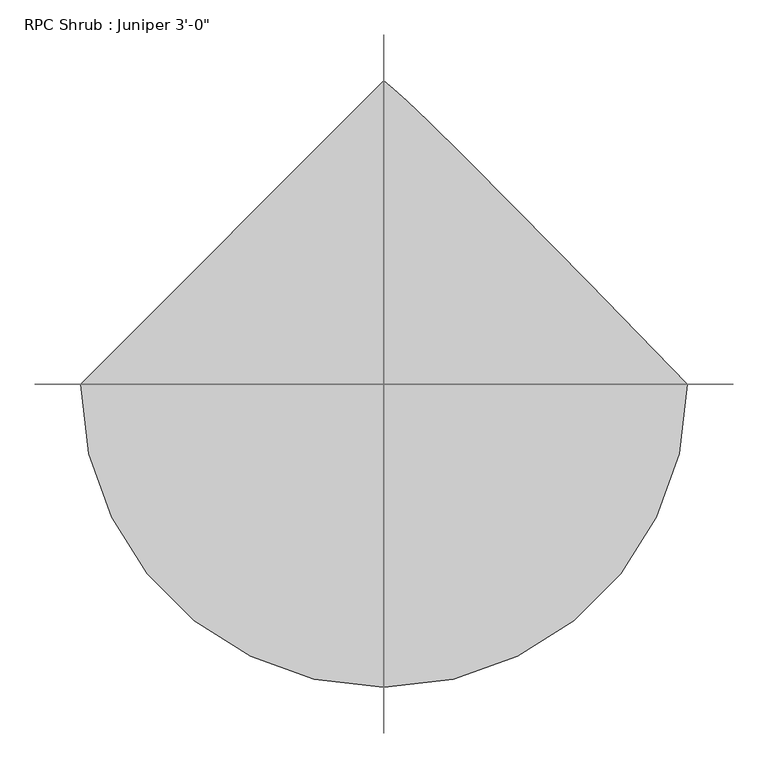
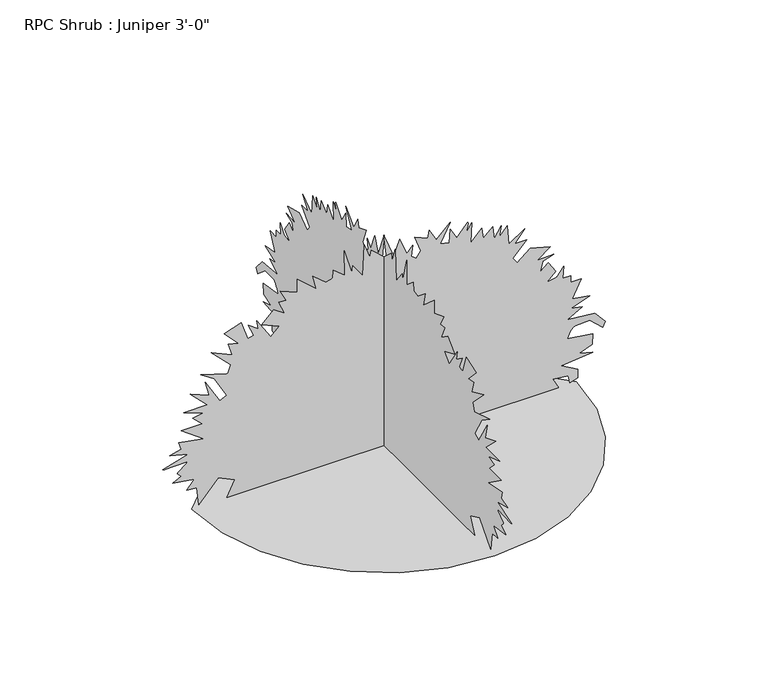
"""IFC4 building model written with IfcOpenShell, lengths in millimetres: geographic element geometry."""

from ifc_helpers import new_model, si_unit, origin, place, context, project, spatial, triangles, source, transform, mapped, element, save


def geographic_element_31b723d7(model_context):
    return source(origin(), model_context, "Body", "Tessellation", [
        triangles([(-789.9406637, 0.0, 7.34e-05), (-769.0593075, -181.0023239, 7.34e-05), (-709.58256, -347.2233553, 7.34e-05), (-616.27561, -493.9033919, 7.34e-05), (-493.9033919, -616.27561, 7.34e-05), (-347.2233553, -709.58256, 7.34e-05), (-181.0023239, -769.0593075, 7.34e-05), (3.45e-05, -789.9406637, 7.34e-05), (181.0025783, -769.0593075, 7.34e-05), (347.2233553, -709.58256, 7.34e-05), (493.9033919, -616.27561, 7.34e-05), (616.27561, -493.9033919, 7.34e-05), (709.58256, -347.2233553, 7.34e-05), (769.0593075, -181.0023239, 7.34e-05), (789.9406637, 6.91e-05, 7.34e-05), (533.2276995, 263.324552, 7.34e-05), (342.9129716, 457.2003633, 7.34e-05), (207.9314215, 593.1996929, 7.34e-05), (117.2157559, 682.8973429, 7.34e-05), (59.6994447, 737.8705862, 7.34e-05), (24.316455, 769.6942978, 7.34e-05), (-0.0001036, 789.9406637, 7.34e-05), (-3.6e-06, -645.975832, 2.9e-06), (1e-06, -614.2334381, 66.8205943), (0.0, -680.8932501, 98.5983058), (0.0, -760.2505428, 9.7171587), (0.0, -769.7755428, 85.9010885), (0.0, -811.0403933, 89.0753315), (0.0, -779.2979994, 127.1672379), (0.0, -868.1777487, 139.8647005), (0.0, -833.2603306, 158.9106491), (0.0, -849.1328356, 174.7823729), (2e-07, -847.0271502, 178.352086), (-1e-07, -810.1082554, 207.9471727), (0.0, -807.8654417, 212.8742702), (2e-07, -903.2958086, 210.5745559), (0.0, -909.4452152, 212.8742702), (0.0, -804.6929609, 244.6174271), (0.0, -880.8752295, 263.6623765), (0.0, -833.2603306, 276.3598392), (0.0, -842.7828598, 308.1047765), (0.0, -741.2056297, 289.0573199), (0.0, -833.2603306, 355.7196754), (0.0, -747.5530621, 355.7196754), (0.0, -785.6455044, 393.8120813), (0.0, -741.2056297, 403.3345379), (0.0, -823.737874, 431.9019439), (0.0, -725.3331247, 431.9019439), (0.0, -795.1679609, 501.7392872), (0.0, -718.9856924, 469.9943499), (0.0, -734.8581247, 533.4817174), (0.0, -674.5432743, 431.9019439), (0.0, -645.975832, 444.5994246), (0.0, -696.7657551, 533.4817174), (0.0, -753.9031105, 571.5741234), (0.0, -642.8008804, 536.6567053), (0.0, -630.1033997, 571.5741234), (0.0, -709.4632359, 650.9314161), (0.0, -623.7558947, 612.8389738), (0.0, -639.6283997, 663.6288969), (0.0, -598.3609694, 654.1063677), (0.0, -655.4982885, 714.4187473), (0.0, -585.663525, 739.8137089), (0.0, -560.2685635, 660.4538727), (0.0, -534.8736382, 666.8038485), (0.0, -557.0935756, 717.5912281), (0.0, -515.8286888, 689.0237858), (6e-07, -522.1761575, 724.2739597), (0.0, -465.0388021, 635.0589111), (0.0, -430.1214203, 669.9763292), (0.0, -503.131208, 701.7212666), (0.0, -452.3413576, 749.3361654), (0.0, -407.901483, 717.5912281), (0.0, -433.2964082, 774.731127), (0.0, -401.5514709, 771.5561028), (0.0, -426.9463961, 819.1710016), (0.0, -357.1115962, 790.6010159), (0.0, -357.1115962, 847.7409147), (0.0, -277.7543035, 777.9035351), (0.0, -293.6242287, 838.2159147), (0.0, -239.6616431, 793.7760401), (0.0, -211.0929654, 800.1260159), (0.0, -207.9182137, 835.043434), (0.0, -160.303333, 796.9510643), (0.0, -163.4780847, 904.8782701), (0.0, -131.7346644, 796.9510643), (0.0, -128.560167, 825.518434), (0.0, -87.2937723, 768.3810785), (0.0, -80.9452954, 901.7032459), (0.0, -58.7248448, 838.2159147), (0.0, -52.3763679, 866.7858278), (0.0, 11.1100709, 809.6484724), (0.0, -1.5869882, 914.4007267), (0.0, 39.6794049, 809.6484724), (0.0, 65.073835, 873.1333328), (0.0, 93.6427671, 800.1260159), (0.0, 119.037447, 828.6934582), (0.0, 112.6887157, 784.2535835), (0.0, 131.7349187, 768.3810785), (0.0, 150.7808674, 793.7760401), (0.0, 125.3861874, 860.4383955), (0.0, 179.3497903, 838.2159147), (0.0, 185.698022, 869.9608521), (0.0, 214.2674628, 819.1710016), (0.0, 271.4042913, 876.308357), (0.0, 230.1389141, 796.9510643), (0.0, 268.2318287, 787.4285351), (0.0, 271.4042913, 844.5658905), (0.0, 299.9742408, 796.9510643), (0.0, 342.3973417, 848.8686802), (0.0, 344.7290671, 848.6756687), (0.0, 345.397086, 844.7309967), (0.0, 338.0666468, 806.4735209), (0.0, 360.2865841, 841.3909389), (0.0, 357.1115962, 755.6835978), (0.0, 401.5540143, 803.2984966), (0.0, 407.901483, 758.858622), (0.0, 445.993889, 793.7760401), (0.0, 452.3413576, 739.8137089), (0.0, 480.9112707, 787.4285351), (0.0, 474.5612949, 739.8137089), (0.0, 506.3062323, 777.9035351), (0.0, 512.6537009, 695.3712908), (0.0, 579.3160563, 739.8137089), (0.0, 538.0486261, 689.0237858), (0.0, 585.663525, 689.0237858), (0.0, 528.5261696, 628.7114788), (0.0, 547.5710827, 603.3165173), (0.0, 601.5359937, 647.7563919), (0.0, 684.0682743, 625.5364546), (0.0, 630.1033997, 584.2716042), (0.0, 696.7657551, 587.4440486), (0.0, 652.3258804, 571.5741234), (0.0, 642.8008804, 530.3066932), (0.0, 674.5458178, 558.8766426), (0.0, 706.2882116, 511.2617801), (0.0, 668.1957693, 476.344362), (0.0, 709.4632359, 482.6918306), (0.0, 738.0306055, 520.7842366), (0.0, 734.8581247, 469.9943499), (0.0, 766.6005186, 469.9943499), (0.0, 766.6005186, 441.4269439), (0.0, 811.0403933, 441.4269439), (0.0, 772.9480236, 368.4171198), (0.0, 845.9578114, 355.7196754), (0.0, 769.7755428, 327.1497259), (0.0, 814.2154175, 317.6272694), (0.0, 753.9031105, 282.7098513), (0.0, 865.0053406, 273.1873765), (0.0, 909.4452152, 222.3972354), (0.0, 899.922686, 200.1767894), (0.0, 845.9578114, 247.7916701), (0.0, 785.3051182, 246.4035645), (0.0, 777.2710882, 242.5165924), (0.0, 770.76618, 236.5473347), (0.0, 765.4803835, 228.9123538), (0.0, 761.1116095, 220.0279215), (0.0, 757.3549347, 210.3106367), (0.0, 753.9031105, 200.1767894), (0.0, 858.6552921, 184.3053381), (0.0, 855.4828114, 139.8647005), (0.0, 801.5179367, 120.8187518), (0.0, 858.6552921, 104.9470462), (0.0, 728.508149, 92.2498288), (0.0, 795.1705044, 54.1576681), (0.0, 795.1705044, 16.0658174), (0.0, 763.4255671, 6.5428419), (0.0, 757.0780621, 38.2862123), (0.0, 693.5907309, 44.6346938), (0.0, 718.9856924, 0.1941814), (-645.975832, 0.000119, 0.0), (-614.2334381, 0.0001104, 66.8205943), (-680.8932501, 0.0001095, 98.5983058), (-760.2505428, 0.0001148, 9.7171587), (-769.7755428, 0.0001102, 85.9010885), (-811.0403933, 0.0001101, 89.0753315), (-779.2979994, 0.0001078, 127.1672379), (-868.1777487, 0.000107, 139.8647005), (-833.2603306, 0.0001059, 158.9106491), (-849.1328356, 0.0001049, 174.7823729), (-847.0271502, 0.0001045, 178.352086), (-810.1082554, 0.000103, 207.9471727), (-807.8654417, 0.0001027, 212.8742702), (-903.2958086, 0.0001026, 210.5745559), (-909.4452152, 0.0001027, 212.8742702), (-804.6929609, 0.0001008, 244.6174271), (-880.8752295, 9.97e-05, 263.6623765), (-833.2603306, 9.89e-05, 276.3598392), (-842.7828598, 9.7e-05, 308.1047765), (-741.2056297, 9.81e-05, 289.0573199), (-833.2603306, 9.42e-05, 355.7196754), (-747.5530621, 9.42e-05, 355.7196754), (-785.6455044, 9.19e-05, 393.8120813), (-741.2056297, 9.13e-05, 403.3345379), (-823.737874, 8.96e-05, 431.9019439), (-725.3331247, 8.96e-05, 431.9019439), (-795.1679609, 8.55e-05, 501.7367437), (-718.9856924, 8.74e-05, 469.9943499), (-734.8581247, 8.36e-05, 533.4817174), (-674.5458178, 8.96e-05, 431.9019439), (-645.975832, 8.89e-05, 444.5994246), (-696.7657551, 8.36e-05, 533.4817174), (-753.9031105, 8.13e-05, 571.5741234), (-642.8008804, 8.34e-05, 536.6567053), (-630.1033997, 8.13e-05, 571.5741234), (-709.4632359, 7.66e-05, 650.9314161), (-623.7558947, 7.88e-05, 612.8389738), (-639.6283997, 7.58e-05, 663.6288969), (-598.3609694, 7.64e-05, 654.1063677), (-655.4982885, 7.28e-05, 714.4187473), (-585.663525, 7.13e-05, 739.8137089), (-560.2685635, 7.6e-05, 660.4538727), (-534.8736382, 7.56e-05, 666.8038485), (-557.0935756, 7.26e-05, 717.5912281), (-515.8286888, 7.43e-05, 689.0237858), (-522.1761575, 7.16e-05, 724.2739597), (-465.0388021, 7.75e-05, 635.0589111), (-430.1214203, 7.54e-05, 669.9763292), (-503.131208, 7.35e-05, 701.7212666), (-452.3413576, 7.07e-05, 749.3361654), (-407.901483, 7.26e-05, 717.5912281), (-433.2964082, 6.92e-05, 774.731127), (-401.5540143, 6.94e-05, 771.5561028), (-426.9463961, 6.65e-05, 819.1710016), (-357.1115962, 6.82e-05, 790.6010159), (-357.1115962, 6.48e-05, 847.7409147), (-277.7543035, 6.9e-05, 777.9035351), (-293.6242287, 6.54e-05, 838.2159147), (-239.6616431, 6.81e-05, 793.7760401), (-211.0929654, 6.77e-05, 800.1260159), (-207.918468, 6.56e-05, 835.043434), (-160.303333, 6.79e-05, 796.9510643), (-163.4780847, 6.14e-05, 904.8782701), (-131.7349187, 6.79e-05, 796.9510643), (-128.560167, 6.62e-05, 825.518434), (-87.2940267, 6.96e-05, 768.3810785), (-80.9452954, 6.16e-05, 901.7032459), (-58.7250992, 6.54e-05, 838.2159147), (-52.3766177, 6.37e-05, 866.7858278), (11.1099687, 6.71e-05, 809.6484724), (-1.5870796, 6.09e-05, 914.4007267), (39.6791505, 6.71e-05, 809.6484724), (65.073835, 6.33e-05, 873.1333328), (93.6427671, 6.77e-05, 800.1260159), (119.037447, 6.6e-05, 828.6934582), (112.6887157, 6.86e-05, 784.2535835), (131.7346644, 6.96e-05, 768.3810785), (150.780613, 6.81e-05, 793.7760401), (125.3861874, 6.41e-05, 860.4358521), (179.349536, 6.54e-05, 838.2159147), (185.698022, 6.35e-05, 869.9608521), (214.2672084, 6.65e-05, 819.1710016), (271.4042913, 6.31e-05, 876.308357), (230.1389141, 6.79e-05, 796.9510643), (268.2318287, 6.84e-05, 787.4285351), (271.4042913, 6.5e-05, 844.5658905), (299.9742408, 6.79e-05, 796.9510643), (342.3973417, 6.48e-05, 848.8686802), (344.7290671, 6.48e-05, 848.6756687), (345.3945425, 6.5e-05, 844.7309967), (338.0666468, 6.73e-05, 806.4735209), (360.2865841, 6.52e-05, 841.3909389), (357.1115962, 7.03e-05, 755.6835978), (401.5514709, 6.75e-05, 803.2984966), (407.901483, 7.01e-05, 758.858622), (445.993889, 6.81e-05, 793.7760401), (452.3413576, 7.13e-05, 739.8137089), (480.9112707, 6.84e-05, 787.4285351), (474.5612949, 7.13e-05, 739.8137089), (506.3062323, 6.9e-05, 777.9035351), (512.6537009, 7.39e-05, 695.3712908), (579.3160563, 7.13e-05, 739.8137089), (538.0486261, 7.43e-05, 689.0237858), (585.663525, 7.43e-05, 689.0237858), (528.5261696, 7.79e-05, 628.7114788), (547.5710827, 7.94e-05, 603.3165173), (601.5359937, 7.68e-05, 647.7563919), (684.0682743, 7.81e-05, 625.5364546), (630.1033997, 8.05e-05, 584.2716042), (696.7657551, 8.04e-05, 587.4440486), (652.3258804, 8.13e-05, 571.5741234), (642.8008804, 8.38e-05, 530.3066932), (674.5458178, 8.21e-05, 558.8766426), (706.2882116, 8.49e-05, 511.2617801), (668.1957693, 8.7e-05, 476.344362), (709.4632359, 8.66e-05, 482.6918306), (738.0306055, 8.43e-05, 520.7842366), (734.8581247, 8.74e-05, 469.9943499), (766.6005186, 8.74e-05, 469.9943499), (766.6005186, 8.91e-05, 441.4269439), (811.0403933, 8.91e-05, 441.4269439), (772.9480236, 9.34e-05, 368.4171198), (845.9578114, 9.42e-05, 355.7196754), (769.7755428, 9.59e-05, 327.1497259), (814.2154175, 9.64e-05, 317.6272694), (753.9031105, 9.85e-05, 282.7098513), (865.0053406, 9.91e-05, 273.1873765), (909.4452152, 0.0001021, 222.3972354), (899.922686, 0.0001034, 200.1767894), (845.9578114, 0.0001006, 247.7916701), (785.3051182, 0.0001007, 246.4035645), (777.2710882, 0.0001009, 242.5165924), (770.76618, 0.0001013, 236.5473347), (765.4803835, 0.0001017, 228.9123538), (761.1116095, 0.0001023, 220.0279215), (757.3549347, 0.0001028, 210.3106367), (753.9031105, 0.0001034, 200.1767894), (858.6552921, 0.0001044, 184.3050838), (855.4828114, 0.000107, 139.8647005), (801.5179367, 0.0001082, 120.8187518), (858.6552921, 0.0001091, 104.9470462), (728.508149, 0.0001099, 92.2495745), (795.1705044, 0.0001121, 54.1576681), (795.1705044, 0.0001144, 16.0658174), (763.4255671, 0.000115, 6.5428419), (757.0780621, 0.0001131, 38.2862123), (693.5907309, 0.0001127, 44.6346938), (718.9856924, 0.0001154, 0.1941786)], [[21, 22, 1], [20, 21, 1], [19, 20, 1], [18, 19, 1], [17, 18, 1], [17, 1, 2], [17, 2, 3], [17, 3, 4], [16, 17, 4], [16, 4, 5], [16, 5, 6], [16, 6, 7], [16, 7, 8], [16, 8, 9], [16, 9, 10], [16, 10, 11], [16, 11, 12], [15, 16, 12], [14, 15, 12], [13, 14, 12], [92, 93, 94], [84, 85, 86], [54, 55, 56], [50, 51, 52], [131, 132, 133], [123, 124, 125], [104, 105, 106], [46, 47, 48], [57, 58, 59], [88, 89, 90], [48, 49, 50], [67, 68, 69], [119, 120, 121], [162, 163, 164], [38, 39, 40], [113, 114, 115], [144, 145, 146], [65, 66, 67], [138, 139, 140], [96, 97, 98], [107, 108, 109], [79, 80, 81], [42, 43, 44], [29, 30, 31], [36, 37, 38], [75, 76, 77], [102, 103, 104], [146, 147, 148], [86, 87, 88], [94, 95, 96], [121, 122, 123], [125, 126, 127], [100, 101, 102], [77, 78, 79], [25, 26, 27], [115, 116, 117], [129, 130, 131], [117, 118, 119], [27, 28, 29], [82, 83, 84], [44, 45, 46], [48, 50, 52], [59, 60, 61], [169, 170, 23], [73, 74, 75], [90, 91, 92], [142, 143, 144], [40, 41, 42], [38, 40, 42], [169, 23, 24], [53, 54, 56], [61, 62, 63], [61, 63, 64], [70, 71, 72], [70, 72, 73], [150, 151, 152], [149, 150, 152], [148, 149, 152], [148, 152, 153], [128, 129, 131], [148, 153, 154], [35, 36, 38], [134, 135, 136], [134, 136, 137], [65, 67, 69], [166, 167, 168], [165, 166, 168], [164, 165, 168], [164, 168, 169], [88, 90, 92], [140, 141, 142], [100, 102, 104], [159, 160, 161], [159, 161, 162], [25, 27, 29], [123, 125, 127], [148, 154, 155], [100, 104, 106], [110, 111, 112], [109, 110, 112], [109, 112, 113], [109, 113, 115], [31, 32, 33], [131, 133, 134], [159, 162, 164], [128, 131, 134], [46, 48, 52], [73, 75, 77], [73, 77, 79], [29, 31, 33], [29, 33, 34], [44, 46, 52], [148, 155, 156], [164, 169, 24], [159, 164, 24], [158, 159, 24], [157, 158, 24], [156, 157, 24], [148, 156, 24], [146, 148, 24], [144, 146, 24], [142, 144, 24], [140, 142, 24], [138, 140, 24], [137, 138, 24], [134, 137, 24], [128, 134, 24], [127, 128, 24], [123, 127, 24], [121, 123, 24], [119, 121, 24], [117, 119, 24], [115, 117, 24], [109, 115, 24], [107, 109, 24], [106, 107, 24], [106, 24, 25], [106, 25, 29], [106, 29, 34], [106, 34, 35], [106, 35, 38], [106, 38, 42], [106, 42, 44], [106, 44, 52], [106, 52, 53], [106, 53, 56], [99, 100, 106], [99, 106, 56], [99, 56, 57], [98, 99, 57], [96, 98, 57], [94, 96, 57], [59, 61, 64], [57, 59, 64], [70, 73, 79], [64, 65, 69], [57, 64, 69], [94, 57, 69], [84, 86, 88], [88, 92, 94], [88, 94, 69], [88, 69, 70], [88, 70, 79], [84, 88, 79], [82, 84, 79], [82, 79, 81], [240, 241, 242], [232, 233, 234], [202, 203, 204], [198, 199, 200], [279, 280, 281], [271, 272, 273], [252, 253, 254], [194, 195, 196], [205, 206, 207], [236, 237, 238], [196, 197, 198], [215, 216, 217], [267, 268, 269], [310, 311, 312], [186, 187, 188], [261, 262, 263], [292, 293, 294], [213, 214, 215], [286, 287, 288], [244, 245, 246], [255, 256, 257], [227, 228, 229], [190, 191, 192], [177, 178, 179], [184, 185, 186], [223, 224, 225], [250, 251, 252], [294, 295, 296], [234, 235, 236], [242, 243, 244], [269, 270, 271], [273, 274, 275], [248, 249, 250], [225, 226, 227], [173, 174, 175], [263, 264, 265], [277, 278, 279], [265, 266, 267], [175, 176, 177], [230, 231, 232], [192, 193, 194], [196, 198, 200], [207, 208, 209], [317, 318, 171], [221, 222, 223], [238, 239, 240], [290, 291, 292], [188, 189, 190], [186, 188, 190], [317, 171, 172], [201, 202, 204], [209, 210, 211], [209, 211, 212], [218, 219, 220], [218, 220, 221], [298, 299, 300], [297, 298, 300], [296, 297, 300], [296, 300, 301], [276, 277, 279], [296, 301, 302], [183, 184, 186], [282, 283, 284], [282, 284, 285], [213, 215, 217], [314, 315, 316], [313, 314, 316], [312, 313, 316], [312, 316, 317], [236, 238, 240], [288, 289, 290], [248, 250, 252], [307, 308, 309], [307, 309, 310], [173, 175, 177], [271, 273, 275], [296, 302, 303], [248, 252, 254], [258, 259, 260], [257, 258, 260], [257, 260, 261], [257, 261, 263], [179, 180, 181], [279, 281, 282], [307, 310, 312], [276, 279, 282], [194, 196, 200], [221, 223, 225], [221, 225, 227], [177, 179, 181], [177, 181, 182], [192, 194, 200], [296, 303, 304], [312, 317, 172], [307, 312, 172], [306, 307, 172], [305, 306, 172], [304, 305, 172], [296, 304, 172], [294, 296, 172], [292, 294, 172], [290, 292, 172], [288, 290, 172], [286, 288, 172], [285, 286, 172], [282, 285, 172], [276, 282, 172], [275, 276, 172], [271, 275, 172], [269, 271, 172], [267, 269, 172], [265, 267, 172], [263, 265, 172], [257, 263, 172], [255, 257, 172], [254, 255, 172], [254, 172, 173], [254, 173, 177], [254, 177, 182], [254, 182, 183], [254, 183, 186], [254, 186, 190], [254, 190, 192], [254, 192, 200], [254, 200, 201], [254, 201, 204], [247, 248, 254], [247, 254, 204], [247, 204, 205], [246, 247, 205], [244, 246, 205], [242, 244, 205], [207, 209, 212], [205, 207, 212], [218, 221, 227], [212, 213, 217], [205, 212, 217], [242, 205, 217], [232, 234, 236], [236, 240, 242], [236, 242, 217], [236, 217, 218], [236, 218, 227], [232, 236, 227], [230, 232, 227], [230, 227, 229]], closed=False),
    ])


if __name__ == "__main__":
    model = new_model("IFC4")
    model_context = context("Model", 3, world=origin())
    ifc_project = project(units=[si_unit("LENGTHUNIT", "METRE", prefix="MILLI")], contexts=[model_context])
    site = spatial("IfcSite", under=ifc_project)
    building = spatial("IfcBuilding", under=site)
    placement = place(None, origin())
    geographic_element_shape = geographic_element_31b723d7(model_context)
    element("IfcGeographicElement", 1, ObjectType="RPC Shrub : Juniper 3'-0\"", at=placement, inside=building, context=model_context, shape_type="MappedRepresentation", body=[
        mapped(geographic_element_shape, transform((0.0, 0.0, 0.0), x_axis=(1.0, 0.0, 0.0), y_axis=(0.0, 1.0, 0.0), z_axis=(0.0, 0.0, 1.0))),
    ])
    save(model, "model.ifc")

# Revit data of these elements
# Type "RPC Shrub : Juniper 3'-0\""
#   Type Comments = "Juniper"
#   built-in parameter 1005198 = "{2, 15},{39, RPC-16-FU4H-UTPX-8HVP-A000-ST1L-LVER-AU},{1, 0},{1, 0},{2, 13},{1, 8},{5, Color},{1, 0},{1, 0},{3, 0.8},{3, 0.8},{3, 0.8},{1, 8},{7, BBoxMin},{1, 0},{1, 0},{1, 0},{1, 0},{1, 0},{1, 8},{7, BBoxMax},{1, 0},{1, 0},{1, 0},{1, 0},{1, 0},{2, 11},{9, RPCTypeId},{1, 0},{1, 0},{39, RPC-16-FU4H-UTPX-8HVP-A000-ST1L-LVER-AU},{1, 6},{14, RPCPlantHeight},{1, 0},{1, 0},{1, 3},{2, 11},{7, keyword},{1, 0},{1, 0},{35, :RPCs:Shrubs & Grasses:Geometry:RPC},{2, 11},{8, category},{1, 0},{1, 0},{16, Shrubs & Grasses},{2, 11},{12, LocalizedUID},{1, 0},{1, 0},{7, Juniper},{2, 14},{6, Height},{1, 0},{1, 0},{1, 3},{1, 2},{16, Cast Reflections},{1, 0},{1, 0},{1, 0},{1, 2},{12, Cast Shadows},{1, 0},{1, 0},{1, 1},{1, 2},{9, Lock View},{1, 0},{1, 0},{1, 0},{1, 4},{5, ViewC},{1, 0},{1, 0},{1, 0},{21, assetlibrary_base.fbx},{1, 5},"
#   built-in parameter 1005195 = "RPC-16-FU4H-UTPX-8HVP-A000-ST1L-LVER-AU"
#   Assembly Code = "G2050500"
#   Height = 3' - 0"
#   Default Elevation = 0
